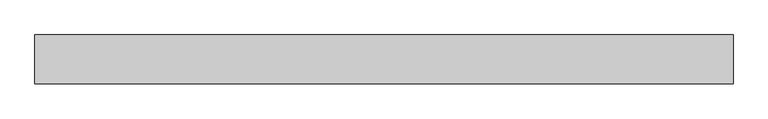
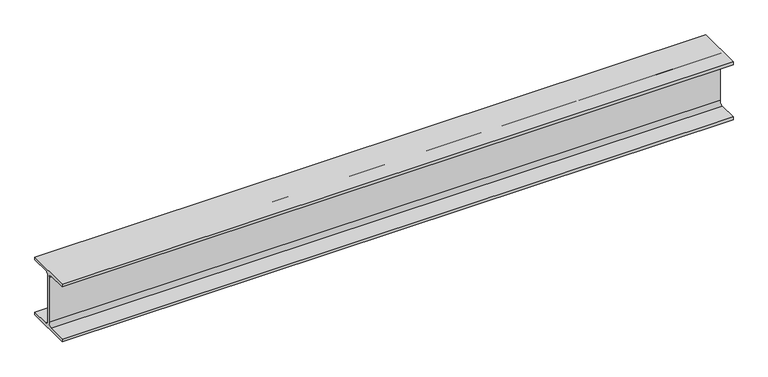
"""IFC4 building model written with IfcOpenShell, lengths in millimetres: beam geometry, 0912_Steel Framing_H-KSD3502 : H_SB_ASB_H-194x150x6x9."""

import ifcopenshell
import ifcopenshell.guid

model = None  # the IFC model being written
_history = None  # IfcOwnerHistory: only IFC2X3 demands one
_inside = {}  # id of a spatial element -> (the spatial element, [elements in it])
_under = {}  # id of a project, library or spatial element -> (it, [spatial elements below it])
_declared = {}  # id of a project -> (the project, [libraries it declares])
_typed = {}  # id of a type object -> (the type object, [elements of that type])
_made_of = {}  # id of a material, layer set ... -> (it, [elements and type objects made of it])


def new_model(schema):
    """Start an empty IFC model of exactly this schema.

    Asked for "IFC4X3", IfcOpenShell would pick the latest addendum, in which some entities
    have other attributes; the version numbers below select the first issue.
    IFC2X3 requires an IfcOwnerHistory on every rooted entity: one is made here for all.
    """
    global model, _history
    if schema == "IFC4X3":
        model = ifcopenshell.file(schema_version=(4, 3, 0, 0))
    else:
        model = ifcopenshell.file(schema=schema)
    _inside.clear()
    _under.clear()
    _declared.clear()
    _typed.clear()
    _made_of.clear()
    _history = None
    if model.schema == "IFC2X3":
        org = make("IfcOrganization", Name="unknown")
        user = make(
            "IfcPersonAndOrganization",
            ThePerson=make("IfcPerson", FamilyName="unknown"),
            TheOrganization=org,
        )
        app = make(
            "IfcApplication",
            ApplicationDeveloper=org,
            Version="unknown",
            ApplicationFullName="unknown",
            ApplicationIdentifier="unknown",
        )
        _history = make(
            "IfcOwnerHistory",
            OwningUser=user,
            OwningApplication=app,
            ChangeAction="ADDED",
            CreationDate=0,
        )
    return model


def make(cls, **values):
    """One entity of the class cls with the attributes given. An attribute that is None is left unset."""
    return model.create_entity(
        cls, **{name: value for name, value in values.items() if value is not None}
    )


def rooted(cls, **values):
    """An entity with a GlobalId (a new one), such as an element, a storey or a relation."""
    return make(cls, GlobalId=ifcopenshell.guid.new(), OwnerHistory=_history, **values)


def si_unit(unit_type, name, prefix=None):
    """IfcSIUnit, for example si_unit("LENGTHUNIT", "METRE", prefix="MILLI")."""
    return make("IfcSIUnit", UnitType=unit_type, Prefix=prefix, Name=name)


def assignment(units):
    """IfcUnitAssignment: the units of a project."""
    return None if units is None else make("IfcUnitAssignment", Units=units)


def point(xyz):
    """IfcCartesianPoint."""
    return None if xyz is None else make("IfcCartesianPoint", Coordinates=xyz)


def direction(xyz):
    """IfcDirection."""
    return None if xyz is None else make("IfcDirection", DirectionRatios=xyz)


def frame(location, z_axis=None, x_axis=None):
    """IfcAxis2Placement3D, a coordinate frame: its origin and axes. An axis left out is left unset."""
    return make(
        "IfcAxis2Placement3D",
        Location=point(location),
        Axis=direction(z_axis),
        RefDirection=direction(x_axis),
    )


def frame_2d(location, x_axis=None):
    """IfcAxis2Placement2D, a coordinate frame in the plane: its origin and x axis."""
    return make(
        "IfcAxis2Placement2D", Location=point(location), RefDirection=direction(x_axis)
    )


def origin():
    """The frame at (0, 0, 0) with its axes left unset."""
    return frame((0.0, 0.0, 0.0))


def place(relative_to, where):
    """IfcLocalPlacement: puts the frame where relative to a parent placement (None: the world)."""
    return make(
        "IfcLocalPlacement", PlacementRelTo=relative_to, RelativePlacement=where
    )


def context(
    kind, dimensions, precision=None, world=None, true_north=None, identifier=None
):
    """IfcGeometricRepresentationContext, for example the 3D "Model" context."""
    return make(
        "IfcGeometricRepresentationContext",
        ContextIdentifier=identifier,
        ContextType=kind,
        CoordinateSpaceDimension=dimensions,
        Precision=precision,
        WorldCoordinateSystem=world,
        TrueNorth=true_north,
    )


def project(units=None, contexts=None):
    """IfcProject with its units and contexts."""
    return rooted(
        "IfcProject",
        Name="project",
        RepresentationContexts=contexts,
        UnitsInContext=assignment(units),
    )


def spatial(cls, under=None, at=None, **own):
    """A site, building, storey or space (cls), placed at a placement, below another one or the project."""
    s = rooted(cls, ObjectPlacement=at, **own)
    if under is not None:
        _under.setdefault(under.id(), (under, []))[1].append(s)
    return s


def polyline(points):
    """IfcPolyline through the points."""
    return make("IfcPolyline", Points=[point(p) for p in points])


def circle_curve(where, radius):
    """IfcCircle in the frame where."""
    return make("IfcCircle", Position=where, Radius=radius)


def trimmed(basis, trim1, trim2, sense, master):
    """IfcTrimmedCurve: the piece of a basis curve between two trims."""
    return make(
        "IfcTrimmedCurve",
        BasisCurve=basis,
        Trim1=trim1,
        Trim2=trim2,
        SenseAgreement=sense,
        MasterRepresentation=master,
    )


def segment(curve, same_sense, transition):
    """IfcCompositeCurveSegment."""
    return make(
        "IfcCompositeCurveSegment",
        Transition=transition,
        SameSense=same_sense,
        ParentCurve=curve,
    )


def composite_curve(segments, self_intersect=None):
    """IfcCompositeCurve: segments joined end to end."""
    return make("IfcCompositeCurve", Segments=segments, SelfIntersect=self_intersect)


def outline(outer, holes=None, kind="AREA"):
    """IfcArbitraryClosedProfileDef: a profile drawn as a closed curve; with holes, ...WithVoids."""
    if holes is None:
        return make("IfcArbitraryClosedProfileDef", ProfileType=kind, OuterCurve=outer)
    return make(
        "IfcArbitraryProfileDefWithVoids",
        ProfileType=kind,
        OuterCurve=outer,
        InnerCurves=holes,
    )


def extrude(swept, where, along, depth):
    """IfcExtrudedAreaSolid: the profile swept, set in the frame where, extruded along a direction by depth."""
    return make(
        "IfcExtrudedAreaSolid",
        SweptArea=swept,
        Position=where,
        ExtrudedDirection=direction(along),
        Depth=depth,
    )


def shape(context_of_items, identifier, shape_type, items):
    """IfcShapeRepresentation: the items that make up one representation, for example the "Body"."""
    return make(
        "IfcShapeRepresentation",
        ContextOfItems=context_of_items,
        RepresentationIdentifier=identifier,
        RepresentationType=shape_type,
        Items=items,
    )


def source(mapping_origin, context_of_items, identifier, shape_type, items):
    """IfcRepresentationMap: a shape defined once, which mapped items show again and again."""
    return make(
        "IfcRepresentationMap",
        MappingOrigin=mapping_origin,
        MappedRepresentation=shape(context_of_items, identifier, shape_type, items),
    )


def transform(
    local_origin,
    x_axis=None,
    y_axis=None,
    z_axis=None,
    scale=None,
    scale2=None,
    scale3=None,
    uniform=True,
):
    """IfcCartesianTransformationOperator3D, or its non-uniform kind. x_axis, y_axis, z_axis: its Axis1, 2, 3."""
    if uniform:
        return make(
            "IfcCartesianTransformationOperator3D",
            Axis1=direction(x_axis),
            Axis2=direction(y_axis),
            LocalOrigin=point(local_origin),
            Scale=scale,
            Axis3=direction(z_axis),
        )
    return make(
        "IfcCartesianTransformationOperator3DnonUniform",
        Axis1=direction(x_axis),
        Axis2=direction(y_axis),
        LocalOrigin=point(local_origin),
        Scale=scale,
        Axis3=direction(z_axis),
        Scale2=scale2,
        Scale3=scale3,
    )


def mapped(mapping_source, mapping_target):
    """IfcMappedItem: shows the shape of a source again, moved by a transform."""
    return make(
        "IfcMappedItem", MappingSource=mapping_source, MappingTarget=mapping_target
    )


def made_of(thing, what):
    """Note that an element or type object is made of a material, layer set ...; save() writes the relation."""
    if what is not None:
        _made_of.setdefault(what.id(), (what, []))[1].append(thing)
    return thing


def element(
    cls,
    number,
    at=None,
    inside=None,
    cuts=None,
    type_object=None,
    material=None,
    context=None,
    identifier="Body",
    shape_type=None,
    held_by="IfcProductDefinitionShape",
    body=None,
    shapes=None,
    **own,
):
    """One element of the class cls, such as IfcWall. Its Tag is "e" and its number.

    at: its placement. inside: the storey or other place that contains it. cuts: it is an
    opening in that element (IfcRelVoidsElement). A single representation is given by context,
    identifier, shape_type and body (its items); several are given by shapes. held_by: the class
    of the entity that holds the representations. save() writes the other relations.
    """
    e = rooted(cls, Tag="e%d" % number, ObjectPlacement=at, **own)
    if body is not None:
        shapes = [shape(context, identifier, shape_type, body)]
    if shapes is not None:
        e.Representation = make(held_by, Representations=shapes)
    if inside is not None:
        _inside.setdefault(inside.id(), (inside, []))[1].append(e)
    if cuts is not None:
        rooted(
            "IfcRelVoidsElement", RelatingBuildingElement=cuts, RelatedOpeningElement=e
        )
    if type_object is not None:
        _typed.setdefault(type_object.id(), (type_object, []))[1].append(e)
    return made_of(e, material)


def aggregate(whole, parts):
    """IfcRelAggregates: a whole, such as a stair, and the parts it consists of."""
    return rooted("IfcRelAggregates", RelatingObject=whole, RelatedObjects=parts)


def save(model, path):
    """Write the relations noted so far, then the file.

    IfcRelAggregates (storeys below a building ...), IfcRelContainedInSpatialStructure (elements
    in a storey), IfcRelDefinesByType, IfcRelAssociatesMaterial and IfcRelDeclares: one each for
    every whole, place, type object, material and project.
    """
    for whole, parts in _under.values():
        aggregate(whole, parts)
    for where, things in _inside.values():
        rooted(
            "IfcRelContainedInSpatialStructure",
            RelatedElements=things,
            RelatingStructure=where,
        )
    for kind, things in _typed.values():
        rooted("IfcRelDefinesByType", RelatedObjects=things, RelatingType=kind)
    for what, things in _made_of.values():
        rooted("IfcRelAssociatesMaterial", RelatedObjects=things, RelatingMaterial=what)
    for by, libraries in _declared.values():
        rooted("IfcRelDeclares", RelatingContext=by, RelatedDefinitions=libraries)
    model.write(path)


def beam_15ee70ce(model_context):
    return source(origin(), model_context, "Body", "SweptSolid", [
        extrude(outline(composite_curve([segment(polyline([(-75.0, -88.0), (-16.0, -88.0)]), True, "CONTINUOUS"), segment(trimmed(circle_curve(frame_2d((-16.0, -75.0)), 13.0), [point((-16.0, -88.0))], [point((-3.0, -75.0))], True, "CARTESIAN"), True, "CONTINUOUS"), segment(polyline([(-3.0, -75.0), (-3.0, 75.0)]), True, "CONTINUOUS"), segment(trimmed(circle_curve(frame_2d((-16.0, 75.0)), 13.0), [point((-3.0, 75.0))], [point((-16.0, 88.0))], True, "CARTESIAN"), True, "CONTINUOUS"), segment(polyline([(-16.0, 88.0), (-75.0, 88.0), (-75.0, 97.0), (75.0, 97.0), (75.0, 88.0), (16.0, 88.0)]), True, "CONTINUOUS"), segment(trimmed(circle_curve(frame_2d((16.0, 75.0)), 13.0), [point((16.0, 88.0))], [point((3.0, 75.0))], True, "CARTESIAN"), True, "CONTINUOUS"), segment(polyline([(3.0, 75.0), (3.0, -75.0)]), True, "CONTINUOUS"), segment(trimmed(circle_curve(frame_2d((16.0, -75.0)), 13.0), [point((3.0, -75.0))], [point((16.0, -88.0))], True, "CARTESIAN"), True, "CONTINUOUS"), segment(polyline([(16.0, -88.0), (75.0, -88.0), (75.0, -97.0), (-75.0, -97.0), (-75.0, -88.0)]), True, "CONTINUOUS")], self_intersect=False)), frame((-1067.7446443, 0.0, 0.0), z_axis=(1.0, 0.0, 0.0), x_axis=(0.0, 1.0, 0.0)), (0.0, 0.0, 1.0), 2135.4892885),
    ])


if __name__ == "__main__":
    model = new_model("IFC4")
    model_context = context("Model", 3, world=origin())
    ifc_project = project(units=[si_unit("LENGTHUNIT", "METRE", prefix="MILLI")], contexts=[model_context])
    site = spatial("IfcSite", under=ifc_project)
    building = spatial("IfcBuilding", under=site)
    placement = place(None, origin())
    beam_shape = beam_15ee70ce(model_context)
    element("IfcBeam", 1, ObjectType="0912_Steel Framing_H-KSD3502 : H_SB_ASB_H-194x150x6x9", at=placement, inside=building, context=model_context, shape_type="MappedRepresentation", body=[
        mapped(beam_shape, transform((0.0, 0.0, 0.0), x_axis=(1.0, 0.0, 0.0), y_axis=(0.0, 1.0, 0.0), z_axis=(0.0, 0.0, 1.0))),
    ])
    save(model, "model.ifc")

# Revit data of these elements
# Type "0912_Steel Framing_H-KSD3502 : H_SB_ASB_H-194x150x6x9"
#   H_WM Code_1 = "S01AA002-00001 | Main Steel Structure Fabrication Work | Shelter/Building | Medium Steel - Standard (90KG/M>Weight≥30KG/M) | Material: (   )"
#   H_WM Code_2 = "S03AA028-00001 | Main Steel Structure Erection Work | Shelter/Building | Medium Steel (90KG/M>Weight≥30KG/M) | Material: (   )"
#   H_WM Code_3 = "S01AA010-00001 | Main Steel Structure Fabrication Work | Shelter/Building | Steel Painting/Coating | for Non-Fireproofed Steel Surface, Surface Preparation, Primer, Second & Final Coat | Material: (   )"
#   H_Q'ty Cal Type Tag = "SB-Q2"
#   Width = 15.0 cm
#   Web Thickness = 0.6 cm
#   Web Fillet = 1.3 cm
#   Warping Constant = 43316.0 cm⁶
#   W = 0
#   Torsional Moment of Inertia = 8.622 cm⁴
#   Section Area = 39.01 cm²
#   Plastic Modulus weak axis = 104.0 cm³
#   Plastic Modulus strong axis = 309.0 cm³
#   Perimeter = 0.95 m²/m
#   Nominal Weight = 30.60 kgf/m
#   Moment of Inertia weak axis = 507.00 cm⁴
#   Moment of Inertia strong axis = 2690.00 cm⁴
#   Height = 19.4 cm
#   Flange Thickness = 0.9 cm
#   Elastic Modulus weak axis = 67.6 cm³
#   Elastic Modulus strong axis = 277.0 cm³
#   Centroid Vertical = 9.7 cm
#   Centroid Horizontal = 7.5 cm
#   Ix = 26900000
#   Length [instance default] = 1.5240 m
#   Zx = 309000
#   b = 0.1500 m
#   h = 0.1940 m
#   r = 0.0130 m
#   s = 0.0060 m
#   t = 0.0090 m
#   A = 0.003901 m²
#   Structural Material [instance default] = Steel, 45-345
#   Assembly Code = ""
# Element 1 (IfcBeam, "0912_Steel Framing_H-KSD3502 : H_SB_ASB_H-194x150x6x9")
#   Structural Material = none
# Materials
#   "Steel, 45-345": class "Metal", colour RGB 189 187 185, transparency 0, Description = "Steel 345 MPa", Cost = 0
